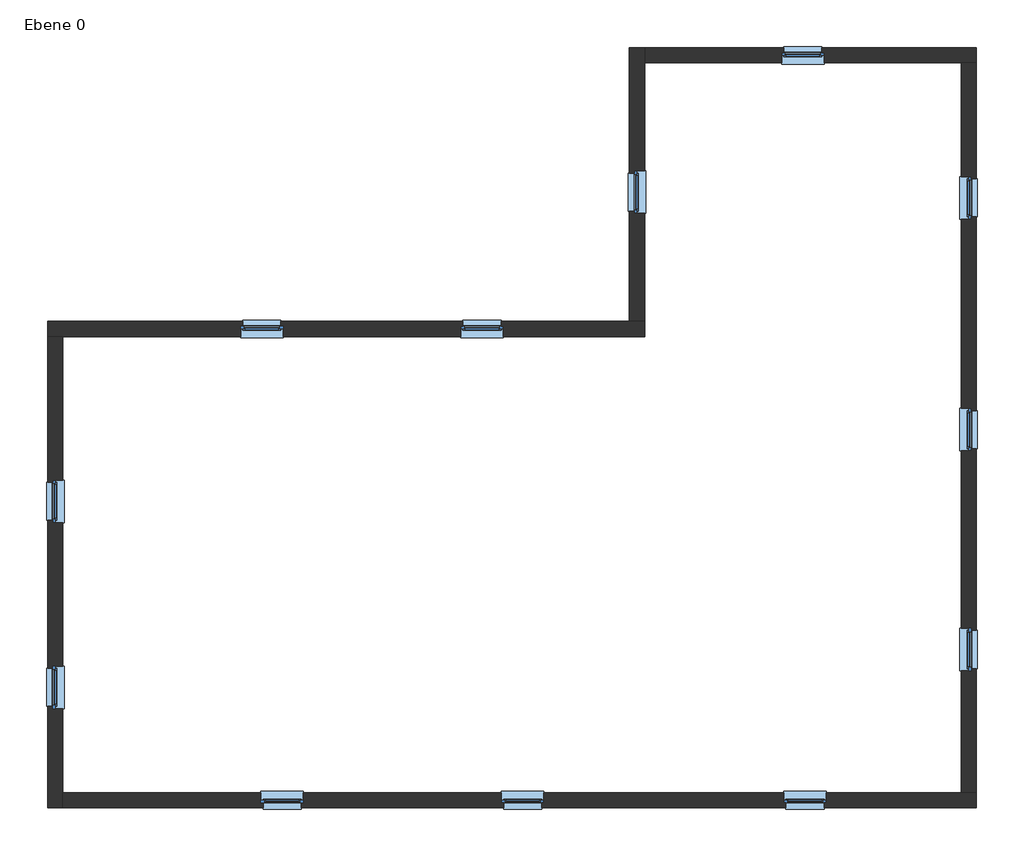
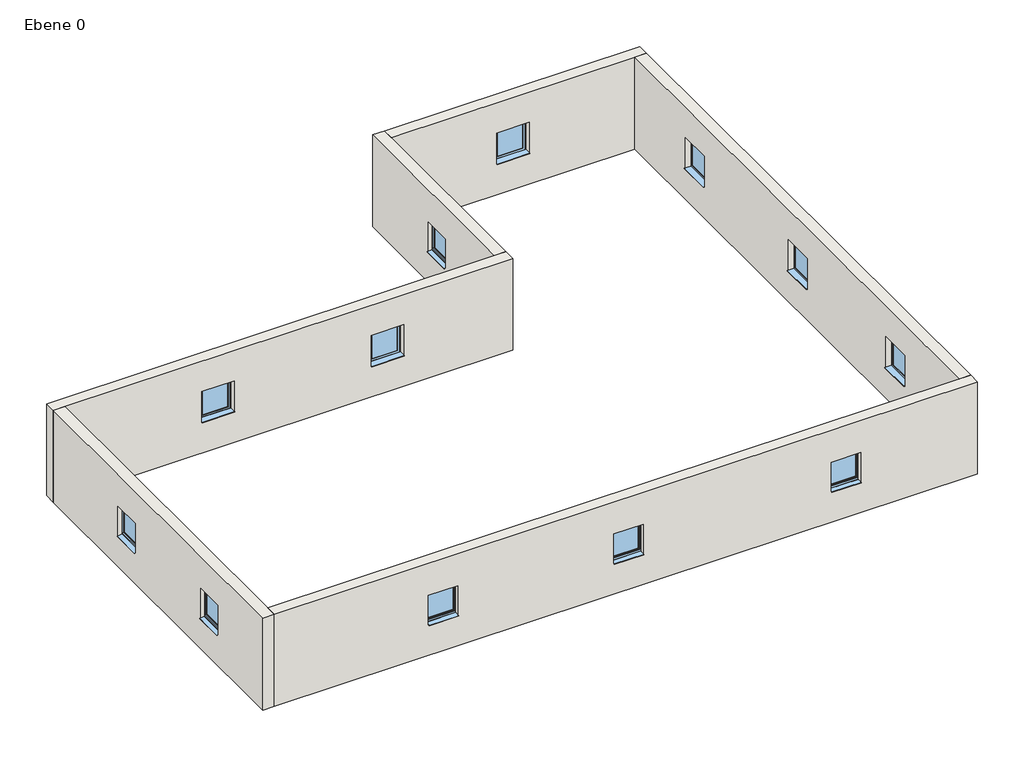
# One storey: 12 windows, 6 walls.
"""IFC4 building model written with IfcOpenShell, lengths in millimetres."""

import ifcopenshell
import ifcopenshell.guid

model = None  # the IFC model being written
_history = None  # IfcOwnerHistory: only IFC2X3 demands one
_inside = {}  # id of a spatial element -> (the spatial element, [elements in it])
_under = {}  # id of a project, library or spatial element -> (it, [spatial elements below it])
_declared = {}  # id of a project -> (the project, [libraries it declares])
_typed = {}  # id of a type object -> (the type object, [elements of that type])
_made_of = {}  # id of a material, layer set ... -> (it, [elements and type objects made of it])


def new_model(schema):
    """Start an empty IFC model of exactly this schema.

    Asked for "IFC4X3", IfcOpenShell would pick the latest addendum, in which some entities
    have other attributes; the version numbers below select the first issue.
    IFC2X3 requires an IfcOwnerHistory on every rooted entity: one is made here for all.
    """
    global model, _history
    if schema == "IFC4X3":
        model = ifcopenshell.file(schema_version=(4, 3, 0, 0))
    else:
        model = ifcopenshell.file(schema=schema)
    _inside.clear()
    _under.clear()
    _declared.clear()
    _typed.clear()
    _made_of.clear()
    _history = None
    if model.schema == "IFC2X3":
        org = make("IfcOrganization", Name="unknown")
        user = make(
            "IfcPersonAndOrganization",
            ThePerson=make("IfcPerson", FamilyName="unknown"),
            TheOrganization=org,
        )
        app = make(
            "IfcApplication",
            ApplicationDeveloper=org,
            Version="unknown",
            ApplicationFullName="unknown",
            ApplicationIdentifier="unknown",
        )
        _history = make(
            "IfcOwnerHistory",
            OwningUser=user,
            OwningApplication=app,
            ChangeAction="ADDED",
            CreationDate=0,
        )
    return model


def make(cls, **values):
    """One entity of the class cls with the attributes given. An attribute that is None is left unset."""
    return model.create_entity(
        cls, **{name: value for name, value in values.items() if value is not None}
    )


def rooted(cls, **values):
    """An entity with a GlobalId (a new one), such as an element, a storey or a relation."""
    return make(cls, GlobalId=ifcopenshell.guid.new(), OwnerHistory=_history, **values)


def si_unit(unit_type, name, prefix=None):
    """IfcSIUnit, for example si_unit("LENGTHUNIT", "METRE", prefix="MILLI")."""
    return make("IfcSIUnit", UnitType=unit_type, Prefix=prefix, Name=name)


def assignment(units):
    """IfcUnitAssignment: the units of a project."""
    return None if units is None else make("IfcUnitAssignment", Units=units)


def point(xyz):
    """IfcCartesianPoint."""
    return None if xyz is None else make("IfcCartesianPoint", Coordinates=xyz)


def direction(xyz):
    """IfcDirection."""
    return None if xyz is None else make("IfcDirection", DirectionRatios=xyz)


def frame(location, z_axis=None, x_axis=None):
    """IfcAxis2Placement3D, a coordinate frame: its origin and axes. An axis left out is left unset."""
    return make(
        "IfcAxis2Placement3D",
        Location=point(location),
        Axis=direction(z_axis),
        RefDirection=direction(x_axis),
    )


def origin():
    """The frame at (0, 0, 0) with its axes left unset."""
    return frame((0.0, 0.0, 0.0))


def place(relative_to, where):
    """IfcLocalPlacement: puts the frame where relative to a parent placement (None: the world)."""
    return make(
        "IfcLocalPlacement", PlacementRelTo=relative_to, RelativePlacement=where
    )


def context(
    kind, dimensions, precision=None, world=None, true_north=None, identifier=None
):
    """IfcGeometricRepresentationContext, for example the 3D "Model" context."""
    return make(
        "IfcGeometricRepresentationContext",
        ContextIdentifier=identifier,
        ContextType=kind,
        CoordinateSpaceDimension=dimensions,
        Precision=precision,
        WorldCoordinateSystem=world,
        TrueNorth=true_north,
    )


def project(units=None, contexts=None):
    """IfcProject with its units and contexts."""
    return rooted(
        "IfcProject",
        Name="project",
        RepresentationContexts=contexts,
        UnitsInContext=assignment(units),
    )


def spatial(cls, under=None, at=None, **own):
    """A site, building, storey or space (cls), placed at a placement, below another one or the project."""
    s = rooted(cls, ObjectPlacement=at, **own)
    if under is not None:
        _under.setdefault(under.id(), (under, []))[1].append(s)
    return s


def polyline(points):
    """IfcPolyline through the points."""
    return make("IfcPolyline", Points=[point(p) for p in points])


def outline(outer, holes=None, kind="AREA"):
    """IfcArbitraryClosedProfileDef: a profile drawn as a closed curve; with holes, ...WithVoids."""
    if holes is None:
        return make("IfcArbitraryClosedProfileDef", ProfileType=kind, OuterCurve=outer)
    return make(
        "IfcArbitraryProfileDefWithVoids",
        ProfileType=kind,
        OuterCurve=outer,
        InnerCurves=holes,
    )


def extrude(swept, where, along, depth):
    """IfcExtrudedAreaSolid: the profile swept, set in the frame where, extruded along a direction by depth."""
    return make(
        "IfcExtrudedAreaSolid",
        SweptArea=swept,
        Position=where,
        ExtrudedDirection=direction(along),
        Depth=depth,
    )


def faces_of(points, faces, orient=None, outer=None):
    """IfcFace entities. A face is a list of loops; a loop is a list of indices into points, from 0.

    orient and outer hold one flag for each loop. By default every Orientation is true, the
    first loop of a face is its IfcFaceOuterBound and the others are IfcFaceBound.
    """
    made = []
    for i, loops in enumerate(faces):
        bounds = []
        for j, loop in enumerate(loops):
            is_outer = j == 0 if outer is None else outer[i][j]
            bounds.append(
                make(
                    "IfcFaceOuterBound" if is_outer else "IfcFaceBound",
                    Bound=make("IfcPolyLoop", Polygon=[points[k] for k in loop]),
                    Orientation=True if orient is None else orient[i][j],
                )
            )
        made.append(make("IfcFace", Bounds=bounds))
    return made


def faceted_brep(points, faces, orient=None, outer=None, voids=None):
    """IfcFacetedBrep: a solid bounded by flat faces; with voids (closed shells), ...WithVoids."""
    shared = [point(p) for p in points]
    hull = make("IfcClosedShell", CfsFaces=faces_of(shared, faces, orient, outer))
    if voids is None:
        return make("IfcFacetedBrep", Outer=hull)
    return make(
        "IfcFacetedBrepWithVoids",
        Outer=hull,
        Voids=[
            make(cls, CfsFaces=faces_of(shared, fs, o, b)) for cls, fs, o, b in voids
        ],
    )


def shape(context_of_items, identifier, shape_type, items):
    """IfcShapeRepresentation: the items that make up one representation, for example the "Body"."""
    return make(
        "IfcShapeRepresentation",
        ContextOfItems=context_of_items,
        RepresentationIdentifier=identifier,
        RepresentationType=shape_type,
        Items=items,
    )


def source(mapping_origin, context_of_items, identifier, shape_type, items):
    """IfcRepresentationMap: a shape defined once, which mapped items show again and again."""
    return make(
        "IfcRepresentationMap",
        MappingOrigin=mapping_origin,
        MappedRepresentation=shape(context_of_items, identifier, shape_type, items),
    )


def transform(
    local_origin,
    x_axis=None,
    y_axis=None,
    z_axis=None,
    scale=None,
    scale2=None,
    scale3=None,
    uniform=True,
):
    """IfcCartesianTransformationOperator3D, or its non-uniform kind. x_axis, y_axis, z_axis: its Axis1, 2, 3."""
    if uniform:
        return make(
            "IfcCartesianTransformationOperator3D",
            Axis1=direction(x_axis),
            Axis2=direction(y_axis),
            LocalOrigin=point(local_origin),
            Scale=scale,
            Axis3=direction(z_axis),
        )
    return make(
        "IfcCartesianTransformationOperator3DnonUniform",
        Axis1=direction(x_axis),
        Axis2=direction(y_axis),
        LocalOrigin=point(local_origin),
        Scale=scale,
        Axis3=direction(z_axis),
        Scale2=scale2,
        Scale3=scale3,
    )


def mapped(mapping_source, mapping_target):
    """IfcMappedItem: shows the shape of a source again, moved by a transform."""
    return make(
        "IfcMappedItem", MappingSource=mapping_source, MappingTarget=mapping_target
    )


def made_of(thing, what):
    """Note that an element or type object is made of a material, layer set ...; save() writes the relation."""
    if what is not None:
        _made_of.setdefault(what.id(), (what, []))[1].append(thing)
    return thing


def element(
    cls,
    number,
    at=None,
    inside=None,
    cuts=None,
    type_object=None,
    material=None,
    context=None,
    identifier="Body",
    shape_type=None,
    held_by="IfcProductDefinitionShape",
    body=None,
    shapes=None,
    **own,
):
    """One element of the class cls, such as IfcWall. Its Tag is "e" and its number.

    at: its placement. inside: the storey or other place that contains it. cuts: it is an
    opening in that element (IfcRelVoidsElement). A single representation is given by context,
    identifier, shape_type and body (its items); several are given by shapes. held_by: the class
    of the entity that holds the representations. save() writes the other relations.
    """
    e = rooted(cls, Tag="e%d" % number, ObjectPlacement=at, **own)
    if body is not None:
        shapes = [shape(context, identifier, shape_type, body)]
    if shapes is not None:
        e.Representation = make(held_by, Representations=shapes)
    if inside is not None:
        _inside.setdefault(inside.id(), (inside, []))[1].append(e)
    if cuts is not None:
        rooted(
            "IfcRelVoidsElement", RelatingBuildingElement=cuts, RelatedOpeningElement=e
        )
    if type_object is not None:
        _typed.setdefault(type_object.id(), (type_object, []))[1].append(e)
    return made_of(e, material)


def aggregate(whole, parts):
    """IfcRelAggregates: a whole, such as a stair, and the parts it consists of."""
    return rooted("IfcRelAggregates", RelatingObject=whole, RelatedObjects=parts)


def save(model, path):
    """Write the relations noted so far, then the file.

    IfcRelAggregates (storeys below a building ...), IfcRelContainedInSpatialStructure (elements
    in a storey), IfcRelDefinesByType, IfcRelAssociatesMaterial and IfcRelDeclares: one each for
    every whole, place, type object, material and project.
    """
    for whole, parts in _under.values():
        aggregate(whole, parts)
    for where, things in _inside.values():
        rooted(
            "IfcRelContainedInSpatialStructure",
            RelatedElements=things,
            RelatingStructure=where,
        )
    for kind, things in _typed.values():
        rooted("IfcRelDefinesByType", RelatedObjects=things, RelatingType=kind)
    for what, things in _made_of.values():
        rooted("IfcRelAssociatesMaterial", RelatedObjects=things, RelatingMaterial=what)
    for by, libraries in _declared.values():
        rooted("IfcRelDeclares", RelatingContext=by, RelatedDefinitions=libraries)
    model.write(path)


def window_1_01_x_1_01_b7243dc8(model_context):
    return source(origin(), model_context, "Body", "SolidModel", [
        extrude(outline(polyline([(-525.0, -210.0), (-525.0, 0.0), (485.0, 0.0), (485.0, -210.0), (-525.0, -210.0)])), frame((0.0, 0.0, 1005.0), z_axis=(0.0, 0.0, 1.0), x_axis=(1.0, 0.0, 0.0)), (0.0, 0.0, 1.0), 15.0),
        extrude(outline(polyline([(375.0, -15.0), (-415.0, -15.0), (-415.0, 15.0), (375.0, 15.0), (375.0, -15.0)])), frame((0.0, 0.0, 1110.0), z_axis=(0.0, 0.0, 1.0), x_axis=(1.0, 0.0, 0.0)), (0.0, 0.0, 1.0), 790.0),
        extrude(outline(polyline([(70.0221543, 1020.0), (210.0, 1000.0), (210.0, 990.0), (208.0, 990.0), (208.0, 998.3604634), (69.8240723, 1018.0), (60.0, 1018.0), (60.0, 1020.0), (70.0221543, 1020.0)])), frame((-475.0, 0.0, 0.0), z_axis=(1.0, 0.0, 0.0), x_axis=(0.0, 1.0, 0.0)), (0.0, 0.0, 1.0), 910.0),
        extrude(outline(polyline([(2010.0, 485.0), (2010.0, -525.0), (1000.0, -525.0), (1000.0, 485.0), (2010.0, 485.0)]), holes=[polyline([(1930.0, 405.0), (1080.0, 405.0), (1080.0, -445.0), (1930.0, -445.0), (1930.0, 405.0)])]), frame((0.0, 0.0, 0.0), z_axis=(0.0, 1.0, 0.0), x_axis=(0.0, 0.0, 1.0)), (0.0, 0.0, 1.0), 60.0),
        faceted_brep([(435.0, 0.0, 1960.0), (435.0, -30.0, 1960.0), (435.0, -30.0, 1050.0), (435.0, 0.0, 1050.0), (-475.0, -30.0, 1960.0), (-475.0, -30.0, 1050.0), (375.0, -30.0, 1110.0), (-415.0, -30.0, 1110.0), (-415.0, -30.0, 1900.0), (375.0, -30.0, 1900.0), (-475.0, 0.0, 1050.0), (-475.0, 0.0, 1960.0), (405.0, 0.0, 1930.0), (-445.0, 0.0, 1930.0), (-445.0, 0.0, 1080.0), (405.0, 0.0, 1080.0), (405.0, 30.0, 1930.0), (405.0, 30.0, 1080.0), (-445.0, 30.0, 1080.0), (-445.0, 30.0, 1930.0), (375.0, 30.0, 1900.0), (-415.0, 30.0, 1900.0), (-415.0, 30.0, 1110.0), (375.0, 30.0, 1110.0)], [[[0, 1, 2, 3]], [[1, 4, 5, 2], [6, 7, 8, 9]], [[3, 2, 5, 10]], [[3, 10, 11, 0], [12, 13, 14, 15]], [[16, 12, 15, 17]], [[17, 15, 14, 18]], [[17, 18, 19, 16], [20, 21, 22, 23]], [[9, 20, 23, 6]], [[6, 23, 22, 7]], [[10, 5, 4, 11]], [[18, 14, 13, 19]], [[7, 22, 21, 8]], [[11, 4, 1, 0]], [[19, 13, 12, 16]], [[8, 21, 20, 9]]]),
    ])


model = new_model("IFC4")

# Units and contexts
model_context = context("Model", 3, world=origin())
ifc_project = project(units=[si_unit("LENGTHUNIT", "METRE", prefix="MILLI")], contexts=[model_context])

# Site, building, storey
site = spatial("IfcSite", under=ifc_project)
building = spatial("IfcBuilding", under=site)
storey = spatial("IfcBuildingStorey", under=building, Name="Ebene 0", Elevation=0.0)

# Walls
placement = place(None, origin())
element("IfcWall", 1, ObjectType="MW 24.0 WD 12.0", at=placement, inside=storey, context=model_context, shape_type="Brep", body=[
    faceted_brep([(-13369.6797169, 6985.6067473, 0.0), (-13009.6797169, 6985.6067473, 0.0), (810.3202831, 6985.6067473, 0.0), (810.3202831, 6985.6067473, 3000.0), (-13009.6797169, 6985.6067473, 3000.0), (-13369.6797169, 6985.6067473, 3000.0), (-2549.6797169, 6985.6067473, 1000.0), (-3559.6797169, 6985.6067473, 1000.0), (-3559.6797169, 6985.6067473, 2010.0), (-2549.6797169, 6985.6067473, 2010.0), (-7779.6797169, 6985.6067473, 1000.0), (-8789.6797169, 6985.6067473, 1000.0), (-8789.6797169, 6985.6067473, 2010.0), (-7779.6797169, 6985.6067473, 2010.0), (-13369.6797169, 7345.6067473, 0.0), (-13369.6797169, 7345.6067473, 3000.0), (450.3202831, 7345.6067473, 3000.0), (810.3202831, 7345.6067473, 3000.0), (810.3202831, 7345.6067473, 0.0), (450.3202831, 7345.6067473, 0.0), (-2599.6797169, 7345.6067473, 1960.0), (-3509.6797169, 7345.6067473, 1960.0), (-3509.6797169, 7345.6067473, 1000.0), (-2599.6797169, 7345.6067473, 1000.0), (-7829.6797169, 7345.6067473, 1960.0), (-8739.6797169, 7345.6067473, 1960.0), (-8739.6797169, 7345.6067473, 1000.0), (-7829.6797169, 7345.6067473, 1000.0), (-2599.6797169, 7225.6067473, 1960.0), (-3509.6797169, 7225.6067473, 1960.0), (-3509.6797169, 7225.6067473, 1000.0), (-2599.6797169, 7225.6067473, 1000.0), (-3559.6797169, 7225.6067473, 1000.0), (-2549.6797169, 7225.6067473, 1000.0), (-3559.6797169, 7225.6067473, 2010.0), (-2549.6797169, 7225.6067473, 2010.0), (-7829.6797169, 7225.6067473, 1960.0), (-8739.6797169, 7225.6067473, 1960.0), (-8739.6797169, 7225.6067473, 1000.0), (-7829.6797169, 7225.6067473, 1000.0), (-8789.6797169, 7225.6067473, 1000.0), (-7779.6797169, 7225.6067473, 1000.0), (-8789.6797169, 7225.6067473, 2010.0), (-7779.6797169, 7225.6067473, 2010.0)], [[[0, 1, 2, 3, 4, 5], [6, 7, 8, 9], [10, 11, 12, 13]], [[14, 15, 16, 17, 18, 19], [20, 21, 22, 23], [24, 25, 26, 27]], [[2, 1, 0, 14, 19, 18]], [[5, 4, 3, 17, 16, 15]], [[0, 5, 15, 14]], [[3, 2, 18, 17]], [[20, 28, 29, 21]], [[21, 29, 30, 22]], [[28, 20, 23, 31]], [[22, 30, 32, 7, 6, 33, 31, 23]], [[34, 35, 9, 8]], [[35, 33, 6, 9]], [[35, 34, 32, 30, 29, 28, 31, 33]], [[32, 34, 8, 7]], [[24, 36, 37, 25]], [[25, 37, 38, 26]], [[36, 24, 27, 39]], [[26, 38, 40, 11, 10, 41, 39, 27]], [[42, 43, 13, 12]], [[43, 41, 10, 13]], [[43, 42, 40, 38, 37, 36, 39, 41]], [[40, 42, 12, 11]]]),
])
element("IfcWall", 2, ObjectType="MW 24.0 WD 12.0", at=placement, inside=storey, context=model_context, shape_type="Brep", body=[
    faceted_brep([(-13009.6797169, -4214.3932527, 0.0), (-13009.6797169, -3854.3932527, 0.0), (-13009.6797169, 6985.6067473, 0.0), (-13009.6797169, 6985.6067473, 3000.0), (-13009.6797169, -3854.3932527, 3000.0), (-13009.6797169, -4214.3932527, 3000.0), (-13009.6797169, -844.3932527, 1000.0), (-13009.6797169, -1854.3932527, 1000.0), (-13009.6797169, -1854.3932527, 2010.0), (-13009.6797169, -844.3932527, 2010.0), (-13009.6797169, 3575.6067473, 1000.0), (-13009.6797169, 2565.6067473, 1000.0), (-13009.6797169, 2565.6067473, 2010.0), (-13009.6797169, 3575.6067473, 2010.0), (-13369.6797169, -4214.3932527, 0.0), (-13369.6797169, -4214.3932527, 3000.0), (-13369.6797169, 6985.6067473, 3000.0), (-13369.6797169, 6985.6067473, 0.0), (-13369.6797169, -894.3932527, 1960.0), (-13369.6797169, -1804.3932527, 1960.0), (-13369.6797169, -1804.3932527, 1000.0), (-13369.6797169, -894.3932527, 1000.0), (-13369.6797169, 3525.6067473, 1960.0), (-13369.6797169, 2615.6067473, 1960.0), (-13369.6797169, 2615.6067473, 1000.0), (-13369.6797169, 3525.6067473, 1000.0), (-13249.6797169, -894.3932527, 1960.0), (-13249.6797169, -1804.3932527, 1960.0), (-13249.6797169, -1804.3932527, 1000.0), (-13249.6797169, -894.3932527, 1000.0), (-13249.6797169, -1854.3932527, 1000.0), (-13249.6797169, -844.3932527, 1000.0), (-13249.6797169, -1854.3932527, 2010.0), (-13249.6797169, -844.3932527, 2010.0), (-13249.6797169, 3525.6067473, 1960.0), (-13249.6797169, 2615.6067473, 1960.0), (-13249.6797169, 2615.6067473, 1000.0), (-13249.6797169, 3525.6067473, 1000.0), (-13249.6797169, 2565.6067473, 1000.0), (-13249.6797169, 3575.6067473, 1000.0), (-13249.6797169, 2565.6067473, 2010.0), (-13249.6797169, 3575.6067473, 2010.0)], [[[0, 1, 2, 3, 4, 5], [6, 7, 8, 9], [10, 11, 12, 13]], [[14, 15, 16, 17], [18, 19, 20, 21], [22, 23, 24, 25]], [[2, 1, 0, 14, 17]], [[5, 4, 3, 16, 15]], [[0, 5, 15, 14]], [[3, 2, 17, 16]], [[18, 26, 27, 19]], [[19, 27, 28, 20]], [[26, 18, 21, 29]], [[20, 28, 30, 7, 6, 31, 29, 21]], [[32, 33, 9, 8]], [[33, 31, 6, 9]], [[33, 32, 30, 28, 27, 26, 29, 31]], [[30, 32, 8, 7]], [[22, 34, 35, 23]], [[23, 35, 36, 24]], [[34, 22, 25, 37]], [[24, 36, 38, 11, 10, 39, 37, 25]], [[40, 41, 13, 12]], [[41, 39, 10, 13]], [[41, 40, 38, 36, 35, 34, 37, 39]], [[38, 40, 12, 11]]]),
])
element("IfcWall", 3, ObjectType="MW 24.0 WD 12.0", at=placement, inside=storey, context=model_context, shape_type="Brep", body=[
    faceted_brep([(8690.3202831, -3854.3932527, 0.0), (8330.3202831, -3854.3932527, 0.0), (-13009.6797169, -3854.3932527, 0.0), (-13009.6797169, -3854.3932527, 3000.0), (8330.3202831, -3854.3932527, 3000.0), (8690.3202831, -3854.3932527, 3000.0), (4120.3202831, -3854.3932527, 1000.0), (5130.3202831, -3854.3932527, 1000.0), (5130.3202831, -3854.3932527, 2010.0), (4120.3202831, -3854.3932527, 2010.0), (-2589.6797169, -3854.3932527, 1000.0), (-1579.6797169, -3854.3932527, 1000.0), (-1579.6797169, -3854.3932527, 2010.0), (-2589.6797169, -3854.3932527, 2010.0), (-8304.6797169, -3854.3932527, 1000.0), (-7294.6797169, -3854.3932527, 1000.0), (-7294.6797169, -3854.3932527, 2010.0), (-8304.6797169, -3854.3932527, 2010.0), (8690.3202831, -4214.3932527, 0.0), (8690.3202831, -4214.3932527, 3000.0), (-13009.6797169, -4214.3932527, 3000.0), (-13009.6797169, -4214.3932527, 0.0), (4170.3202831, -4214.3932527, 1960.0), (5080.3202831, -4214.3932527, 1960.0), (5080.3202831, -4214.3932527, 1000.0), (4170.3202831, -4214.3932527, 1000.0), (-2539.6797169, -4214.3932527, 1960.0), (-1629.6797169, -4214.3932527, 1960.0), (-1629.6797169, -4214.3932527, 1000.0), (-2539.6797169, -4214.3932527, 1000.0), (-8254.6797169, -4214.3932527, 1960.0), (-7344.6797169, -4214.3932527, 1960.0), (-7344.6797169, -4214.3932527, 1000.0), (-8254.6797169, -4214.3932527, 1000.0), (4170.3202831, -4094.3932527, 1960.0), (5080.3202831, -4094.3932527, 1960.0), (5080.3202831, -4094.3932527, 1000.0), (4170.3202831, -4094.3932527, 1000.0), (5130.3202831, -4094.3932527, 1000.0), (4120.3202831, -4094.3932527, 1000.0), (5130.3202831, -4094.3932527, 2010.0), (4120.3202831, -4094.3932527, 2010.0), (-2539.6797169, -4094.3932527, 1960.0), (-1629.6797169, -4094.3932527, 1960.0), (-1629.6797169, -4094.3932527, 1000.0), (-2539.6797169, -4094.3932527, 1000.0), (-1579.6797169, -4094.3932527, 1000.0), (-2589.6797169, -4094.3932527, 1000.0), (-1579.6797169, -4094.3932527, 2010.0), (-2589.6797169, -4094.3932527, 2010.0), (-8254.6797169, -4094.3932527, 1960.0), (-7344.6797169, -4094.3932527, 1960.0), (-7344.6797169, -4094.3932527, 1000.0), (-8254.6797169, -4094.3932527, 1000.0), (-7294.6797169, -4094.3932527, 1000.0), (-8304.6797169, -4094.3932527, 1000.0), (-7294.6797169, -4094.3932527, 2010.0), (-8304.6797169, -4094.3932527, 2010.0)], [[[0, 1, 2, 3, 4, 5], [6, 7, 8, 9], [10, 11, 12, 13], [14, 15, 16, 17]], [[18, 19, 20, 21], [22, 23, 24, 25], [26, 27, 28, 29], [30, 31, 32, 33]], [[2, 1, 0, 18, 21]], [[5, 4, 3, 20, 19]], [[0, 5, 19, 18]], [[3, 2, 21, 20]], [[22, 34, 35, 23]], [[23, 35, 36, 24]], [[34, 22, 25, 37]], [[24, 36, 38, 7, 6, 39, 37, 25]], [[40, 41, 9, 8]], [[41, 39, 6, 9]], [[41, 40, 38, 36, 35, 34, 37, 39]], [[38, 40, 8, 7]], [[26, 42, 43, 27]], [[27, 43, 44, 28]], [[42, 26, 29, 45]], [[28, 44, 46, 11, 10, 47, 45, 29]], [[48, 49, 13, 12]], [[49, 47, 10, 13]], [[49, 48, 46, 44, 43, 42, 45, 47]], [[46, 48, 12, 11]], [[30, 50, 51, 31]], [[31, 51, 52, 32]], [[50, 30, 33, 53]], [[32, 52, 54, 15, 14, 55, 53, 33]], [[56, 57, 17, 16]], [[57, 55, 14, 17]], [[57, 56, 54, 52, 51, 50, 53, 55]], [[54, 56, 16, 15]]]),
])
element("IfcWall", 4, ObjectType="MW 24.0 WD 12.0", at=placement, inside=storey, context=model_context, shape_type="Brep", body=[
    faceted_brep([(8330.3202831, 13485.6067473, 0.0), (8330.3202831, -3854.3932527, 0.0), (8330.3202831, -3854.3932527, 3000.0), (8330.3202831, 13485.6067473, 3000.0), (8330.3202831, 9775.6067473, 1000.0), (8330.3202831, 10785.6067473, 1000.0), (8330.3202831, 10785.6067473, 2010.0), (8330.3202831, 9775.6067473, 2010.0), (8330.3202831, 4265.6067473, 1000.0), (8330.3202831, 5275.6067473, 1000.0), (8330.3202831, 5275.6067473, 2010.0), (8330.3202831, 4265.6067473, 2010.0), (8330.3202831, -954.3932527, 1000.0), (8330.3202831, 55.6067473, 1000.0), (8330.3202831, 55.6067473, 2010.0), (8330.3202831, -954.3932527, 2010.0), (8690.3202831, 13485.6067473, 0.0), (8690.3202831, 13485.6067473, 3000.0), (8690.3202831, -3854.3932527, 3000.0), (8690.3202831, -3854.3932527, 0.0), (8690.3202831, 9825.6067473, 1960.0), (8690.3202831, 10735.6067473, 1960.0), (8690.3202831, 10735.6067473, 1000.0), (8690.3202831, 9825.6067473, 1000.0), (8690.3202831, 4315.6067473, 1960.0), (8690.3202831, 5225.6067473, 1960.0), (8690.3202831, 5225.6067473, 1000.0), (8690.3202831, 4315.6067473, 1000.0), (8690.3202831, -904.3932527, 1960.0), (8690.3202831, 5.6067473, 1960.0), (8690.3202831, 5.6067473, 1000.0), (8690.3202831, -904.3932527, 1000.0), (8570.3202831, 9825.6067473, 1960.0), (8570.3202831, 10735.6067473, 1960.0), (8570.3202831, 10735.6067473, 1000.0), (8570.3202831, 9825.6067473, 1000.0), (8570.3202831, 10785.6067473, 1000.0), (8570.3202831, 9775.6067473, 1000.0), (8570.3202831, 10785.6067473, 2010.0), (8570.3202831, 9775.6067473, 2010.0), (8570.3202831, 4315.6067473, 1960.0), (8570.3202831, 5225.6067473, 1960.0), (8570.3202831, 5225.6067473, 1000.0), (8570.3202831, 4315.6067473, 1000.0), (8570.3202831, 5275.6067473, 1000.0), (8570.3202831, 4265.6067473, 1000.0), (8570.3202831, 5275.6067473, 2010.0), (8570.3202831, 4265.6067473, 2010.0), (8570.3202831, -904.3932527, 1960.0), (8570.3202831, 5.6067473, 1960.0), (8570.3202831, 5.6067473, 1000.0), (8570.3202831, -904.3932527, 1000.0), (8570.3202831, 55.6067473, 1000.0), (8570.3202831, -954.3932527, 1000.0), (8570.3202831, 55.6067473, 2010.0), (8570.3202831, -954.3932527, 2010.0)], [[[0, 1, 2, 3], [4, 5, 6, 7], [8, 9, 10, 11], [12, 13, 14, 15]], [[16, 17, 18, 19], [20, 21, 22, 23], [24, 25, 26, 27], [28, 29, 30, 31]], [[1, 0, 16, 19]], [[3, 2, 18, 17]], [[2, 1, 19, 18]], [[0, 3, 17, 16]], [[20, 32, 33, 21]], [[21, 33, 34, 22]], [[32, 20, 23, 35]], [[22, 34, 36, 5, 4, 37, 35, 23]], [[38, 39, 7, 6]], [[39, 37, 4, 7]], [[39, 38, 36, 34, 33, 32, 35, 37]], [[36, 38, 6, 5]], [[24, 40, 41, 25]], [[25, 41, 42, 26]], [[40, 24, 27, 43]], [[26, 42, 44, 9, 8, 45, 43, 27]], [[46, 47, 11, 10]], [[47, 45, 8, 11]], [[47, 46, 44, 42, 41, 40, 43, 45]], [[44, 46, 10, 9]], [[28, 48, 49, 29]], [[29, 49, 50, 30]], [[48, 28, 31, 51]], [[30, 50, 52, 13, 12, 53, 51, 31]], [[54, 55, 15, 14]], [[55, 53, 12, 15]], [[55, 54, 52, 50, 49, 48, 51, 53]], [[52, 54, 14, 13]]]),
])
element("IfcWall", 5, ObjectType="MW 24.0 WD 12.0", at=placement, inside=storey, context=model_context, shape_type="Brep", body=[
    faceted_brep([(810.3202831, 7345.6067473, 0.0), (810.3202831, 13485.6067473, 0.0), (810.3202831, 13845.6067473, 0.0), (810.3202831, 13845.6067473, 3000.0), (810.3202831, 13485.6067473, 3000.0), (810.3202831, 7345.6067473, 3000.0), (810.3202831, 10920.6067473, 1000.0), (810.3202831, 9910.6067473, 1000.0), (810.3202831, 9910.6067473, 2010.0), (810.3202831, 10920.6067473, 2010.0), (450.3202831, 7345.6067473, 0.0), (450.3202831, 7345.6067473, 3000.0), (450.3202831, 13845.6067473, 3000.0), (450.3202831, 13845.6067473, 0.0), (450.3202831, 10870.6067473, 1960.0), (450.3202831, 9960.6067473, 1960.0), (450.3202831, 9960.6067473, 1000.0), (450.3202831, 10870.6067473, 1000.0), (570.3202831, 10870.6067473, 1960.0), (570.3202831, 9960.6067473, 1960.0), (570.3202831, 9960.6067473, 1000.0), (570.3202831, 10870.6067473, 1000.0), (570.3202831, 9910.6067473, 1000.0), (570.3202831, 10920.6067473, 1000.0), (570.3202831, 9910.6067473, 2010.0), (570.3202831, 10920.6067473, 2010.0)], [[[0, 1, 2, 3, 4, 5], [6, 7, 8, 9]], [[10, 11, 12, 13], [14, 15, 16, 17]], [[2, 1, 0, 10, 13]], [[5, 4, 3, 12, 11]], [[3, 2, 13, 12]], [[0, 5, 11, 10]], [[14, 18, 19, 15]], [[15, 19, 20, 16]], [[18, 14, 17, 21]], [[16, 20, 22, 7, 6, 23, 21, 17]], [[24, 25, 9, 8]], [[25, 23, 6, 9]], [[25, 24, 22, 20, 19, 18, 21, 23]], [[22, 24, 8, 7]]]),
])
element("IfcWall", 6, ObjectType="MW 24.0 WD 12.0", at=placement, inside=storey, context=model_context, shape_type="Brep", body=[
    faceted_brep([(810.3202831, 13485.6067473, 0.0), (8330.3202831, 13485.6067473, 0.0), (8690.3202831, 13485.6067473, 0.0), (8690.3202831, 13485.6067473, 3000.0), (8330.3202831, 13485.6067473, 3000.0), (810.3202831, 13485.6067473, 3000.0), (5075.3202831, 13485.6067473, 1000.0), (4065.3202831, 13485.6067473, 1000.0), (4065.3202831, 13485.6067473, 2010.0), (5075.3202831, 13485.6067473, 2010.0), (810.3202831, 13845.6067473, 0.0), (810.3202831, 13845.6067473, 3000.0), (8690.3202831, 13845.6067473, 3000.0), (8690.3202831, 13845.6067473, 0.0), (5025.3202831, 13845.6067473, 1960.0), (4115.3202831, 13845.6067473, 1960.0), (4115.3202831, 13845.6067473, 1000.0), (5025.3202831, 13845.6067473, 1000.0), (5025.3202831, 13725.6067473, 1960.0), (4115.3202831, 13725.6067473, 1960.0), (4115.3202831, 13725.6067473, 1000.0), (5025.3202831, 13725.6067473, 1000.0), (4065.3202831, 13725.6067473, 1000.0), (5075.3202831, 13725.6067473, 1000.0), (4065.3202831, 13725.6067473, 2010.0), (5075.3202831, 13725.6067473, 2010.0)], [[[0, 1, 2, 3, 4, 5], [6, 7, 8, 9]], [[10, 11, 12, 13], [14, 15, 16, 17]], [[2, 1, 0, 10, 13]], [[5, 4, 3, 12, 11]], [[0, 5, 11, 10]], [[3, 2, 13, 12]], [[14, 18, 19, 15]], [[15, 19, 20, 16]], [[18, 14, 17, 21]], [[16, 20, 22, 7, 6, 23, 21, 17]], [[24, 25, 9, 8]], [[25, 23, 6, 9]], [[25, 24, 22, 20, 19, 18, 21, 23]], [[22, 24, 8, 7]]]),
])

# Windows
window_1_01_x_1_01_shape = window_1_01_x_1_01_b7243dc8(model_context)
element("IfcWindow", 7, ObjectType="Fenster 1-flg - Anschlag : 1.01 x 1.01", at=placement, inside=storey, context=model_context, shape_type="MappedRepresentation", body=[
    mapped(window_1_01_x_1_01_shape, transform((4590.3202831, 13665.6067473, 0.0), x_axis=(1.0, 0.0, 0.0), y_axis=(0.0, 1.0, 0.0), z_axis=(0.0, 0.0, 1.0))),
])
element("IfcWindow", 8, ObjectType="Fenster 1-flg - Anschlag : 1.01 x 1.01", at=placement, inside=storey, context=model_context, shape_type="MappedRepresentation", body=[
    mapped(window_1_01_x_1_01_shape, transform((630.3202831, 10435.6067473, 0.0), x_axis=(0.0, 1.0, 0.0), y_axis=(-1.0, 0.0, 0.0), z_axis=(0.0, 0.0, 1.0))),
])
element("IfcWindow", 9, ObjectType="Fenster 1-flg - Anschlag : 1.01 x 1.01", at=placement, inside=storey, context=model_context, shape_type="MappedRepresentation", body=[
    mapped(window_1_01_x_1_01_shape, transform((-3034.6797169, 7165.6067473, 0.0), x_axis=(1.0, 0.0, 0.0), y_axis=(0.0, 1.0, 0.0), z_axis=(0.0, 0.0, 1.0))),
])
element("IfcWindow", 10, ObjectType="Fenster 1-flg - Anschlag : 1.01 x 1.01", at=placement, inside=storey, context=model_context, shape_type="MappedRepresentation", body=[
    mapped(window_1_01_x_1_01_shape, transform((-8264.6797169, 7165.6067473, 0.0), x_axis=(1.0, 0.0, 0.0), y_axis=(0.0, 1.0, 0.0), z_axis=(0.0, 0.0, 1.0))),
])
element("IfcWindow", 11, ObjectType="Fenster 1-flg - Anschlag : 1.01 x 1.01", at=placement, inside=storey, context=model_context, shape_type="MappedRepresentation", body=[
    mapped(window_1_01_x_1_01_shape, transform((8510.3202831, 10260.6067473, 0.0), x_axis=(0.0, -1.0, 0.0), y_axis=(1.0, 0.0, 0.0), z_axis=(0.0, 0.0, 1.0))),
])
element("IfcWindow", 12, ObjectType="Fenster 1-flg - Anschlag : 1.01 x 1.01", at=placement, inside=storey, context=model_context, shape_type="MappedRepresentation", body=[
    mapped(window_1_01_x_1_01_shape, transform((8510.3202831, 4750.6067473, 0.0), x_axis=(0.0, -1.0, 0.0), y_axis=(1.0, 0.0, 0.0), z_axis=(0.0, 0.0, 1.0))),
])
element("IfcWindow", 13, ObjectType="Fenster 1-flg - Anschlag : 1.01 x 1.01", at=placement, inside=storey, context=model_context, shape_type="MappedRepresentation", body=[
    mapped(window_1_01_x_1_01_shape, transform((8510.3202831, -469.3932527, 0.0), x_axis=(0.0, -1.0, 0.0), y_axis=(1.0, 0.0, 0.0), z_axis=(0.0, 0.0, 1.0))),
])
element("IfcWindow", 14, ObjectType="Fenster 1-flg - Anschlag : 1.01 x 1.01", at=placement, inside=storey, context=model_context, shape_type="MappedRepresentation", body=[
    mapped(window_1_01_x_1_01_shape, transform((4605.3202831, -4034.3932527, 0.0), x_axis=(-1.0, 0.0, 0.0), y_axis=(0.0, -1.0, 0.0), z_axis=(0.0, 0.0, 1.0))),
])
element("IfcWindow", 15, ObjectType="Fenster 1-flg - Anschlag : 1.01 x 1.01", at=placement, inside=storey, context=model_context, shape_type="MappedRepresentation", body=[
    mapped(window_1_01_x_1_01_shape, transform((-2104.6797169, -4034.3932527, 0.0), x_axis=(-1.0, 0.0, 0.0), y_axis=(0.0, -1.0, 0.0), z_axis=(0.0, 0.0, 1.0))),
])
element("IfcWindow", 16, ObjectType="Fenster 1-flg - Anschlag : 1.01 x 1.01", at=placement, inside=storey, context=model_context, shape_type="MappedRepresentation", body=[
    mapped(window_1_01_x_1_01_shape, transform((-7819.6797169, -4034.3932527, 0.0), x_axis=(-1.0, 0.0, 0.0), y_axis=(0.0, -1.0, 0.0), z_axis=(0.0, 0.0, 1.0))),
])
element("IfcWindow", 17, ObjectType="Fenster 1-flg - Anschlag : 1.01 x 1.01", at=placement, inside=storey, context=model_context, shape_type="MappedRepresentation", body=[
    mapped(window_1_01_x_1_01_shape, transform((-13189.6797169, -1329.3932527, 0.0), x_axis=(0.0, 1.0, 0.0), y_axis=(-1.0, 0.0, 0.0), z_axis=(0.0, 0.0, 1.0))),
])
element("IfcWindow", 18, ObjectType="Fenster 1-flg - Anschlag : 1.01 x 1.01", at=placement, inside=storey, context=model_context, shape_type="MappedRepresentation", body=[
    mapped(window_1_01_x_1_01_shape, transform((-13189.6797169, 3090.6067473, 0.0), x_axis=(0.0, 1.0, 0.0), y_axis=(-1.0, 0.0, 0.0), z_axis=(0.0, 0.0, 1.0))),
])

save(model, "model.ifc")

# Revit data of these elements
# Project information
#   Projektausgabedatum = "Projekt Datum"
#   Projektstatus = "Projektstatus"
#   Kundenname = "Bauherr"
#   Projektadresse = "Projektadresse"
#   Projektname = "Projektname"
#   Projektnummer = "Projektnummer"
#   Verfasser Firma 1 = "Firma 1"
#   Verfasser Firma 2 = "Firma 2"
#   Verfasser PLZ Ort = "PLZ Ort"
#   Verfasser Strasse = "Strasse"
#   Verfasser Telefon = "Telefon"
#   Verfasser Telefax = "Telefax"
#   Verfasser eMail = "E-Mail"
# Type "MW 24.0 WD 12.0"
#   Type Comments = "Mehrschaliges Mauerwerk"
#   Description = "Mauerwerk 24.0 cm, Wärmedämmung 12.0 cm"
#   Width = 0.360 m
#   Layers, outside or top first: 0.120 m "Wärmedämmung - Hart" (function 3); 0.240 m "Mauerwerk - Ziegel, verputzt" (function 1)
# Type "Fenster 1-flg - Anschlag : 1.01 x 1.01"
#   Type Mark = "47"
#   Operation = "SinglePanel"
#   Keynote = "16.05.01"
#   Construction Type Id = "GSP4R"
#   Analytic Construction = "1/8 Zoll Pilkington-Verglasung einfach"
#   Visual Light Transmittance = 0.9
#   Thermal Resistance (R) = 0.1491 (m²·K)/W
#   Solar Heat Gain Coefficient = 0.86
#   Anschlagsbreite seitlich = 0.050 m
#   Rough Width = 1.010 m
#   Rough Height = 1.010 m
#   Heat Transfer Coefficient (U) = 6.7069 W/(m²·K)
#   Rahmentiefe = 0.060 m
#   Rahmenhöhe unten = 0.080 m
#   Rahmenhöhe oben = 0.080 m
#   Rahmenbreite = 0.080 m
#   Height = 1.010 m
#   Flügeltiefe = 0.060 m
#   Flügelbreite = 0.060 m
#   Einbautiefe (von außen) [instance default] = 0.120 m
#   Width = 1.010 m
#   Anschlagsbreite oben = 0.050 m
#   Klappflügel [instance default] = no
#   Öffnungsrichtung oben [instance default] = yes
#   Öffnungsrichtung in Draufsicht anzeigen [instance default] = no
#   Drehflügel [instance default] = yes
#   Rahmen [instance default] = none
#   Glas [instance default] = none
#   Flügel [instance default] = none
#   Fensterbank innen [instance default] = none
#   Fensterbank außen [instance default] = none
#   Wall Closure = (empty or 0)
# Elements 1, 4 (IfcWall, "MW 24.0 WD 12.0")
#   Top Offset = 0.000 m
#   Base Offset = 0.000 m
#   wall height = 3.000 m
#   Phase Created = Phase 1
#   Base Constraint = Ebene 0
#   Top Constraint = Ebene 1
#   Materials on its faces: "Standard - Wand", "Mauerwerk - Ziegel, verputzt", "Wärmedämmung - Hart"
# Elements 2, 3, 5, 6 (IfcWall, "MW 24.0 WD 12.0")
#   Top Offset = 0.000 m
#   Base Offset = 0.000 m
#   wall height = 3.000 m
#   Phase Created = Phase 1
#   Base Constraint = Ebene 0
#   Top Constraint = Ebene 1
#   Materials on its faces: "Standard - Wand", "Wärmedämmung - Hart", "Mauerwerk - Ziegel, verputzt"
# Element 7 (IfcWindow, "Fenster 1-flg - Anschlag : 1.01 x 1.01")
#   Mark = "1"
#   Einbautiefe (von außen) = 0.120 m
#   Öffnungsrichtung oben = yes
#   Öffnungsrichtung in Draufsicht anzeigen = no
#   Klappflügel = no
#   Drehflügel = yes
#   Rahmen = none
#   Glas = none
#   Flügel = none
#   Fensterbank innen = none
#   Fensterbank außen = none
#   Phase Created = Phase 1
#   Materials on its faces: "Kunststoff - Weiß", "Holz - Birke", "Glas"
# Element 8 (IfcWindow, "Fenster 1-flg - Anschlag : 1.01 x 1.01")
#   Mark = "2"
#   Einbautiefe (von außen) = 0.120 m
#   Öffnungsrichtung oben = yes
#   Öffnungsrichtung in Draufsicht anzeigen = no
#   Klappflügel = no
#   Drehflügel = yes
#   Rahmen = none
#   Glas = none
#   Flügel = none
#   Fensterbank innen = none
#   Fensterbank außen = none
#   Phase Created = Phase 1
#   Materials on its faces: "Kunststoff - Weiß", "Holz - Birke", "Glas"
# Element 9 (IfcWindow, "Fenster 1-flg - Anschlag : 1.01 x 1.01")
#   Mark = "3"
#   Einbautiefe (von außen) = 0.120 m
#   Öffnungsrichtung oben = yes
#   Öffnungsrichtung in Draufsicht anzeigen = no
#   Klappflügel = no
#   Drehflügel = yes
#   Rahmen = none
#   Glas = none
#   Flügel = none
#   Fensterbank innen = none
#   Fensterbank außen = none
#   Phase Created = Phase 1
#   Materials on its faces: "Kunststoff - Weiß", "Holz - Birke", "Glas"
# Element 10 (IfcWindow, "Fenster 1-flg - Anschlag : 1.01 x 1.01")
#   Mark = "4"
#   Einbautiefe (von außen) = 0.120 m
#   Öffnungsrichtung oben = yes
#   Öffnungsrichtung in Draufsicht anzeigen = no
#   Klappflügel = no
#   Drehflügel = yes
#   Rahmen = none
#   Glas = none
#   Flügel = none
#   Fensterbank innen = none
#   Fensterbank außen = none
#   Phase Created = Phase 1
#   Materials on its faces: "Kunststoff - Weiß", "Holz - Birke", "Glas"
# Element 11 (IfcWindow, "Fenster 1-flg - Anschlag : 1.01 x 1.01")
#   Mark = "5"
#   Einbautiefe (von außen) = 0.120 m
#   Öffnungsrichtung oben = yes
#   Öffnungsrichtung in Draufsicht anzeigen = no
#   Klappflügel = no
#   Drehflügel = yes
#   Rahmen = none
#   Glas = none
#   Flügel = none
#   Fensterbank innen = none
#   Fensterbank außen = none
#   Phase Created = Phase 1
#   Materials on its faces: "Kunststoff - Weiß", "Holz - Birke", "Glas"
# Element 12 (IfcWindow, "Fenster 1-flg - Anschlag : 1.01 x 1.01")
#   Mark = "6"
#   Einbautiefe (von außen) = 0.120 m
#   Öffnungsrichtung oben = yes
#   Öffnungsrichtung in Draufsicht anzeigen = no
#   Klappflügel = no
#   Drehflügel = yes
#   Rahmen = none
#   Glas = none
#   Flügel = none
#   Fensterbank innen = none
#   Fensterbank außen = none
#   Phase Created = Phase 1
#   Materials on its faces: "Kunststoff - Weiß", "Holz - Birke", "Glas"
# Element 13 (IfcWindow, "Fenster 1-flg - Anschlag : 1.01 x 1.01")
#   Mark = "7"
#   Einbautiefe (von außen) = 0.120 m
#   Öffnungsrichtung oben = yes
#   Öffnungsrichtung in Draufsicht anzeigen = no
#   Klappflügel = no
#   Drehflügel = yes
#   Rahmen = none
#   Glas = none
#   Flügel = none
#   Fensterbank innen = none
#   Fensterbank außen = none
#   Phase Created = Phase 1
#   Materials on its faces: "Kunststoff - Weiß", "Holz - Birke", "Glas"
# Element 14 (IfcWindow, "Fenster 1-flg - Anschlag : 1.01 x 1.01")
#   Mark = "8"
#   Einbautiefe (von außen) = 0.120 m
#   Öffnungsrichtung oben = yes
#   Öffnungsrichtung in Draufsicht anzeigen = no
#   Klappflügel = no
#   Drehflügel = yes
#   Rahmen = none
#   Glas = none
#   Flügel = none
#   Fensterbank innen = none
#   Fensterbank außen = none
#   Phase Created = Phase 1
#   Materials on its faces: "Kunststoff - Weiß", "Holz - Birke", "Glas"
# Element 15 (IfcWindow, "Fenster 1-flg - Anschlag : 1.01 x 1.01")
#   Mark = "9"
#   Einbautiefe (von außen) = 0.120 m
#   Öffnungsrichtung oben = yes
#   Öffnungsrichtung in Draufsicht anzeigen = no
#   Klappflügel = no
#   Drehflügel = yes
#   Rahmen = none
#   Glas = none
#   Flügel = none
#   Fensterbank innen = none
#   Fensterbank außen = none
#   Phase Created = Phase 1
#   Materials on its faces: "Kunststoff - Weiß", "Holz - Birke", "Glas"
# Element 16 (IfcWindow, "Fenster 1-flg - Anschlag : 1.01 x 1.01")
#   Mark = "10"
#   Einbautiefe (von außen) = 0.120 m
#   Öffnungsrichtung oben = yes
#   Öffnungsrichtung in Draufsicht anzeigen = no
#   Klappflügel = no
#   Drehflügel = yes
#   Rahmen = none
#   Glas = none
#   Flügel = none
#   Fensterbank innen = none
#   Fensterbank außen = none
#   Phase Created = Phase 1
#   Materials on its faces: "Kunststoff - Weiß", "Holz - Birke", "Glas"
# Element 17 (IfcWindow, "Fenster 1-flg - Anschlag : 1.01 x 1.01")
#   Mark = "11"
#   Einbautiefe (von außen) = 0.120 m
#   Öffnungsrichtung oben = yes
#   Öffnungsrichtung in Draufsicht anzeigen = no
#   Klappflügel = no
#   Drehflügel = yes
#   Rahmen = none
#   Glas = none
#   Flügel = none
#   Fensterbank innen = none
#   Fensterbank außen = none
#   Phase Created = Phase 1
#   Materials on its faces: "Kunststoff - Weiß", "Holz - Birke", "Glas"
# Element 18 (IfcWindow, "Fenster 1-flg - Anschlag : 1.01 x 1.01")
#   Mark = "12"
#   Einbautiefe (von außen) = 0.120 m
#   Öffnungsrichtung oben = yes
#   Öffnungsrichtung in Draufsicht anzeigen = no
#   Klappflügel = no
#   Drehflügel = yes
#   Rahmen = none
#   Glas = none
#   Flügel = none
#   Fensterbank innen = none
#   Fensterbank außen = none
#   Phase Created = Phase 1
#   Materials on its faces: "Kunststoff - Weiß", "Holz - Birke", "Glas"
# Materials
#   "Wärmedämmung - Hart": class "Putz", colour RGB 255 255 255, transparency 0, Description = "Äußere Oberfläche"
#   "Mauerwerk - Ziegel, verputzt": class "Putz", colour RGB 247 247 247, transparency 0, Cost = 0
#   "Standard - Wand": class "Putz", colour RGB 128 128 128, transparency 0, Description = "Äußere Oberfläche"
#   "Kunststoff - Weiß": class "Kunststoff", colour RGB 249 249 249, transparency 0
#   "Holz - Birke": class "Holz", colour RGB 213 164 103, transparency 0
#   "Glas": class "Glas", colour RGB 0 0 255, transparency 0.75, Comments = "Renderdarstellung nicht aktualisiert ", Cost = 0
